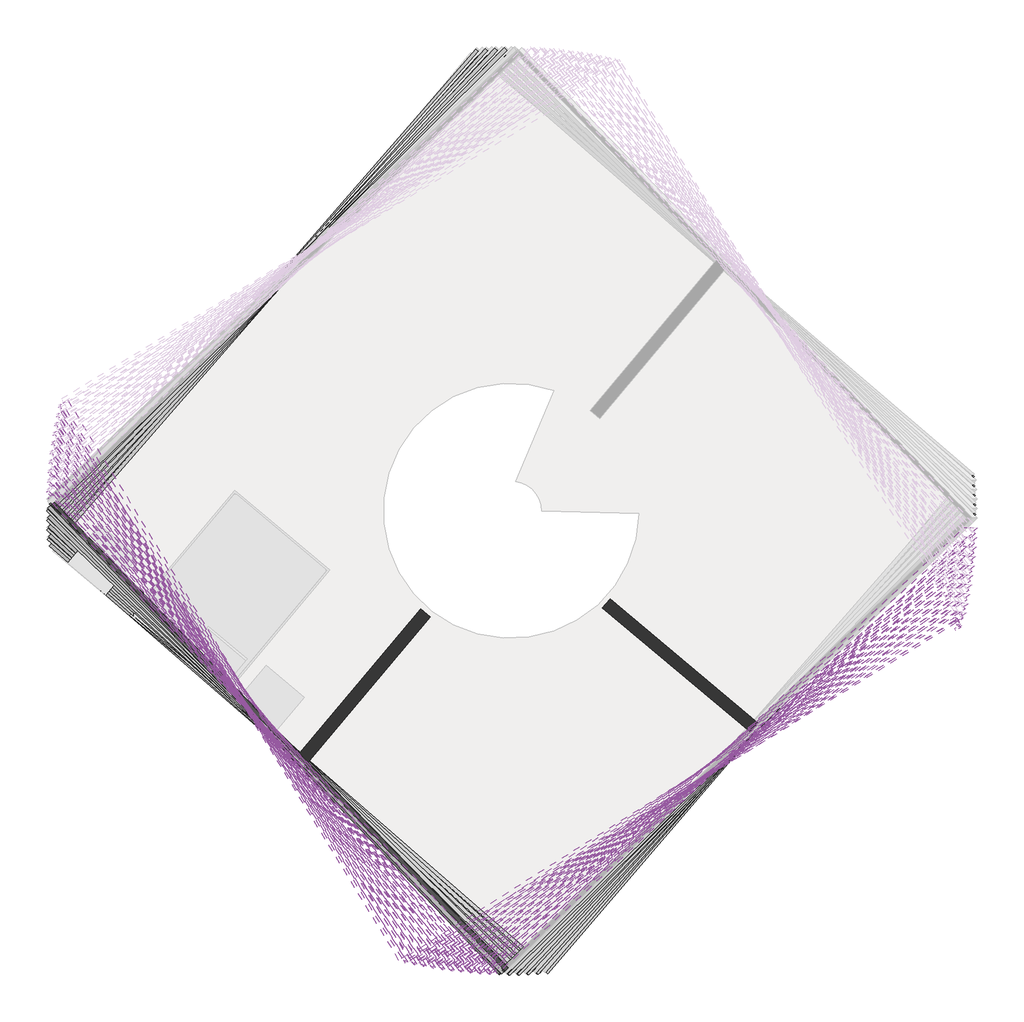
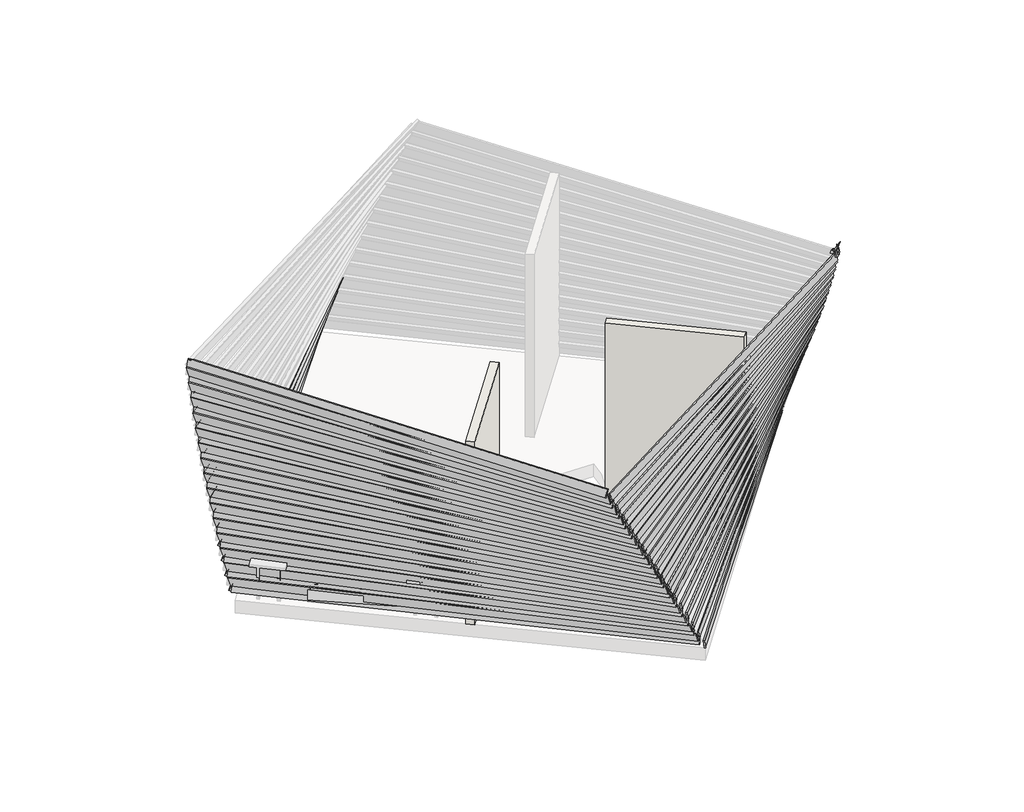
# One storey, part 1 of 2: 33 plates, 32 members, 2 walls.
"""IFC4 building model written with IfcOpenShell, lengths in millimetres."""

import ifcopenshell
import ifcopenshell.guid

model = None  # the IFC model being written
_history = None  # IfcOwnerHistory: only IFC2X3 demands one
_inside = {}  # id of a spatial element -> (the spatial element, [elements in it])
_under = {}  # id of a project, library or spatial element -> (it, [spatial elements below it])
_declared = {}  # id of a project -> (the project, [libraries it declares])
_typed = {}  # id of a type object -> (the type object, [elements of that type])
_made_of = {}  # id of a material, layer set ... -> (it, [elements and type objects made of it])


def new_model(schema):
    """Start an empty IFC model of exactly this schema.

    Asked for "IFC4X3", IfcOpenShell would pick the latest addendum, in which some entities
    have other attributes; the version numbers below select the first issue.
    IFC2X3 requires an IfcOwnerHistory on every rooted entity: one is made here for all.
    """
    global model, _history
    if schema == "IFC4X3":
        model = ifcopenshell.file(schema_version=(4, 3, 0, 0))
    else:
        model = ifcopenshell.file(schema=schema)
    _inside.clear()
    _under.clear()
    _declared.clear()
    _typed.clear()
    _made_of.clear()
    _history = None
    if model.schema == "IFC2X3":
        org = make("IfcOrganization", Name="unknown")
        user = make(
            "IfcPersonAndOrganization",
            ThePerson=make("IfcPerson", FamilyName="unknown"),
            TheOrganization=org,
        )
        app = make(
            "IfcApplication",
            ApplicationDeveloper=org,
            Version="unknown",
            ApplicationFullName="unknown",
            ApplicationIdentifier="unknown",
        )
        _history = make(
            "IfcOwnerHistory",
            OwningUser=user,
            OwningApplication=app,
            ChangeAction="ADDED",
            CreationDate=0,
        )
    return model


def make(cls, **values):
    """One entity of the class cls with the attributes given. An attribute that is None is left unset."""
    return model.create_entity(
        cls, **{name: value for name, value in values.items() if value is not None}
    )


def rooted(cls, **values):
    """An entity with a GlobalId (a new one), such as an element, a storey or a relation."""
    return make(cls, GlobalId=ifcopenshell.guid.new(), OwnerHistory=_history, **values)


def si_unit(unit_type, name, prefix=None):
    """IfcSIUnit, for example si_unit("LENGTHUNIT", "METRE", prefix="MILLI")."""
    return make("IfcSIUnit", UnitType=unit_type, Prefix=prefix, Name=name)


def assignment(units):
    """IfcUnitAssignment: the units of a project."""
    return None if units is None else make("IfcUnitAssignment", Units=units)


def point(xyz):
    """IfcCartesianPoint."""
    return None if xyz is None else make("IfcCartesianPoint", Coordinates=xyz)


def direction(xyz):
    """IfcDirection."""
    return None if xyz is None else make("IfcDirection", DirectionRatios=xyz)


def frame(location, z_axis=None, x_axis=None):
    """IfcAxis2Placement3D, a coordinate frame: its origin and axes. An axis left out is left unset."""
    return make(
        "IfcAxis2Placement3D",
        Location=point(location),
        Axis=direction(z_axis),
        RefDirection=direction(x_axis),
    )


def origin():
    """The frame at (0, 0, 0) with its axes left unset."""
    return frame((0.0, 0.0, 0.0))


def place(relative_to, where):
    """IfcLocalPlacement: puts the frame where relative to a parent placement (None: the world)."""
    return make(
        "IfcLocalPlacement", PlacementRelTo=relative_to, RelativePlacement=where
    )


def context(
    kind, dimensions, precision=None, world=None, true_north=None, identifier=None
):
    """IfcGeometricRepresentationContext, for example the 3D "Model" context."""
    return make(
        "IfcGeometricRepresentationContext",
        ContextIdentifier=identifier,
        ContextType=kind,
        CoordinateSpaceDimension=dimensions,
        Precision=precision,
        WorldCoordinateSystem=world,
        TrueNorth=true_north,
    )


def project(units=None, contexts=None):
    """IfcProject with its units and contexts."""
    return rooted(
        "IfcProject",
        Name="project",
        RepresentationContexts=contexts,
        UnitsInContext=assignment(units),
    )


def spatial(cls, under=None, at=None, **own):
    """A site, building, storey or space (cls), placed at a placement, below another one or the project."""
    s = rooted(cls, ObjectPlacement=at, **own)
    if under is not None:
        _under.setdefault(under.id(), (under, []))[1].append(s)
    return s


def polyline(points):
    """IfcPolyline through the points."""
    return make("IfcPolyline", Points=[point(p) for p in points])


def outline(outer, holes=None, kind="AREA"):
    """IfcArbitraryClosedProfileDef: a profile drawn as a closed curve; with holes, ...WithVoids."""
    if holes is None:
        return make("IfcArbitraryClosedProfileDef", ProfileType=kind, OuterCurve=outer)
    return make(
        "IfcArbitraryProfileDefWithVoids",
        ProfileType=kind,
        OuterCurve=outer,
        InnerCurves=holes,
    )


def extrude(swept, where, along, depth):
    """IfcExtrudedAreaSolid: the profile swept, set in the frame where, extruded along a direction by depth."""
    return make(
        "IfcExtrudedAreaSolid",
        SweptArea=swept,
        Position=where,
        ExtrudedDirection=direction(along),
        Depth=depth,
    )


def faces_of(points, faces, orient=None, outer=None):
    """IfcFace entities. A face is a list of loops; a loop is a list of indices into points, from 0.

    orient and outer hold one flag for each loop. By default every Orientation is true, the
    first loop of a face is its IfcFaceOuterBound and the others are IfcFaceBound.
    """
    made = []
    for i, loops in enumerate(faces):
        bounds = []
        for j, loop in enumerate(loops):
            is_outer = j == 0 if outer is None else outer[i][j]
            bounds.append(
                make(
                    "IfcFaceOuterBound" if is_outer else "IfcFaceBound",
                    Bound=make("IfcPolyLoop", Polygon=[points[k] for k in loop]),
                    Orientation=True if orient is None else orient[i][j],
                )
            )
        made.append(make("IfcFace", Bounds=bounds))
    return made


def faceted_brep(points, faces, orient=None, outer=None, voids=None):
    """IfcFacetedBrep: a solid bounded by flat faces; with voids (closed shells), ...WithVoids."""
    shared = [point(p) for p in points]
    hull = make("IfcClosedShell", CfsFaces=faces_of(shared, faces, orient, outer))
    if voids is None:
        return make("IfcFacetedBrep", Outer=hull)
    return make(
        "IfcFacetedBrepWithVoids",
        Outer=hull,
        Voids=[
            make(cls, CfsFaces=faces_of(shared, fs, o, b)) for cls, fs, o, b in voids
        ],
    )


def shape(context_of_items, identifier, shape_type, items):
    """IfcShapeRepresentation: the items that make up one representation, for example the "Body"."""
    return make(
        "IfcShapeRepresentation",
        ContextOfItems=context_of_items,
        RepresentationIdentifier=identifier,
        RepresentationType=shape_type,
        Items=items,
    )


def source(mapping_origin, context_of_items, identifier, shape_type, items):
    """IfcRepresentationMap: a shape defined once, which mapped items show again and again."""
    return make(
        "IfcRepresentationMap",
        MappingOrigin=mapping_origin,
        MappedRepresentation=shape(context_of_items, identifier, shape_type, items),
    )


def transform(
    local_origin,
    x_axis=None,
    y_axis=None,
    z_axis=None,
    scale=None,
    scale2=None,
    scale3=None,
    uniform=True,
):
    """IfcCartesianTransformationOperator3D, or its non-uniform kind. x_axis, y_axis, z_axis: its Axis1, 2, 3."""
    if uniform:
        return make(
            "IfcCartesianTransformationOperator3D",
            Axis1=direction(x_axis),
            Axis2=direction(y_axis),
            LocalOrigin=point(local_origin),
            Scale=scale,
            Axis3=direction(z_axis),
        )
    return make(
        "IfcCartesianTransformationOperator3DnonUniform",
        Axis1=direction(x_axis),
        Axis2=direction(y_axis),
        LocalOrigin=point(local_origin),
        Scale=scale,
        Axis3=direction(z_axis),
        Scale2=scale2,
        Scale3=scale3,
    )


def mapped(mapping_source, mapping_target):
    """IfcMappedItem: shows the shape of a source again, moved by a transform."""
    return make(
        "IfcMappedItem", MappingSource=mapping_source, MappingTarget=mapping_target
    )


def made_of(thing, what):
    """Note that an element or type object is made of a material, layer set ...; save() writes the relation."""
    if what is not None:
        _made_of.setdefault(what.id(), (what, []))[1].append(thing)
    return thing


def element(
    cls,
    number,
    at=None,
    inside=None,
    cuts=None,
    type_object=None,
    material=None,
    context=None,
    identifier="Body",
    shape_type=None,
    held_by="IfcProductDefinitionShape",
    body=None,
    shapes=None,
    **own,
):
    """One element of the class cls, such as IfcWall. Its Tag is "e" and its number.

    at: its placement. inside: the storey or other place that contains it. cuts: it is an
    opening in that element (IfcRelVoidsElement). A single representation is given by context,
    identifier, shape_type and body (its items); several are given by shapes. held_by: the class
    of the entity that holds the representations. save() writes the other relations.
    """
    e = rooted(cls, Tag="e%d" % number, ObjectPlacement=at, **own)
    if body is not None:
        shapes = [shape(context, identifier, shape_type, body)]
    if shapes is not None:
        e.Representation = make(held_by, Representations=shapes)
    if inside is not None:
        _inside.setdefault(inside.id(), (inside, []))[1].append(e)
    if cuts is not None:
        rooted(
            "IfcRelVoidsElement", RelatingBuildingElement=cuts, RelatedOpeningElement=e
        )
    if type_object is not None:
        _typed.setdefault(type_object.id(), (type_object, []))[1].append(e)
    return made_of(e, material)


def aggregate(whole, parts):
    """IfcRelAggregates: a whole, such as a stair, and the parts it consists of."""
    return rooted("IfcRelAggregates", RelatingObject=whole, RelatedObjects=parts)


def save(model, path):
    """Write the relations noted so far, then the file.

    IfcRelAggregates (storeys below a building ...), IfcRelContainedInSpatialStructure (elements
    in a storey), IfcRelDefinesByType, IfcRelAssociatesMaterial and IfcRelDeclares: one each for
    every whole, place, type object, material and project.
    """
    for whole, parts in _under.values():
        aggregate(whole, parts)
    for where, things in _inside.values():
        rooted(
            "IfcRelContainedInSpatialStructure",
            RelatedElements=things,
            RelatingStructure=where,
        )
    for kind, things in _typed.values():
        rooted("IfcRelDefinesByType", RelatedObjects=things, RelatingType=kind)
    for what, things in _made_of.values():
        rooted("IfcRelAssociatesMaterial", RelatedObjects=things, RelatingMaterial=what)
    for by, libraries in _declared.values():
        rooted("IfcRelDeclares", RelatingContext=by, RelatedDefinitions=libraries)
    model.write(path)


def rectangular_mullion_0e496170(model_context):
    return source(origin(), model_context, "Body", "SweptSolid", [
        extrude(outline(polyline([(-35.3553391, 70.7106781), (70.7106781, -35.3553391), (35.3553391, -70.7106781), (-70.7106781, 35.3553391), (-35.3553391, 70.7106781)])), frame((0.0, 0.0, -8000.0002611), z_axis=(0.0, 0.0, 1.0), x_axis=(1.0, 0.0, 0.0)), (0.0, 0.0, 1.0), 8000.0002611),
    ])


def rectangular_mullion_04c84a83(model_context):
    return source(origin(), model_context, "Body", "SweptSolid", [
        extrude(outline(polyline([(-35.3553391, 70.7106781), (70.7106781, -35.3553391), (35.3553391, -70.7106781), (-70.7106781, 35.3553391), (-35.3553391, 70.7106781)])), frame((0.0, 0.0, -7999.7790849), z_axis=(0.0, 0.0, 1.0), x_axis=(1.0, 0.0, 0.0)), (0.0, 0.0, 1.0), 7999.7790849),
    ])


def rectangular_mullion_5ffb7332(model_context):
    return source(origin(), model_context, "Body", "SweptSolid", [
        extrude(outline(polyline([(-35.3553391, 70.7106781), (70.7106781, -35.3553391), (35.3553391, -70.7106781), (-70.7106781, 35.3553391), (-35.3553391, 70.7106781)])), frame((0.0, 0.0, -7999.4864286), z_axis=(0.0, 0.0, 1.0), x_axis=(1.0, 0.0, 0.0)), (0.0, 0.0, 1.0), 7999.4864286),
    ])


def rectangular_mullion_42344c31(model_context):
    return source(origin(), model_context, "Body", "SweptSolid", [
        extrude(outline(polyline([(-35.3553391, 70.7106781), (70.7106781, -35.3553391), (35.3553391, -70.7106781), (-70.7106781, 35.3553391), (-35.3553391, 70.7106781)])), frame((0.0, 0.0, -7999.2546449), z_axis=(0.0, 0.0, 1.0), x_axis=(1.0, 0.0, 0.0)), (0.0, 0.0, 1.0), 7999.2546449),
    ])


def rectangular_mullion_749d1d03(model_context):
    return source(origin(), model_context, "Body", "Brep", [
        faceted_brep([(-35.3553391, 70.7106781, -7999.1607688), (70.7106781, -35.3553391, -7999.1607688), (35.3553391, -70.7106781, -7999.1607688), (-70.7106781, 35.3553391, -7999.1607688), (-70.7106781, 35.3553391, 10.0516542), (-35.3553391, 70.7106781, 55.0905224), (35.3553391, -70.7106781, -55.0905224), (70.7106781, -35.3553391, -10.0516542)], [[[0, 1, 2, 3]], [[4, 5, 0, 3]], [[6, 4, 3, 2]], [[7, 6, 2, 1]], [[5, 7, 1, 0]], [[5, 4, 6, 7]]]),
    ])


def rectangular_mullion_bea0bdf5(model_context):
    return source(origin(), model_context, "Body", "Brep", [
        faceted_brep([(-35.3553391, 70.7106781, -7999.3358332), (70.7106781, -35.3553391, -7999.3358332), (35.3553391, -70.7106781, -7999.3358332), (-70.7106781, 35.3553391, -7999.3358332), (-70.7106781, 35.3553391, 10.0090632), (-35.3553391, 70.7106781, 55.0597182), (35.3553391, -70.7106781, -55.0597182), (70.7106781, -35.3553391, -10.0090632)], [[[0, 1, 2, 3]], [[4, 5, 0, 3]], [[6, 4, 3, 2]], [[7, 6, 2, 1]], [[5, 7, 1, 0]], [[5, 4, 6, 7]]]),
    ])


def rectangular_mullion_7177dd57(model_context):
    return source(origin(), model_context, "Body", "Brep", [
        faceted_brep([(-35.3553391, 70.7106781, -7999.2401644), (70.7106781, -35.3553391, -7999.2401644), (35.3553391, -70.7106781, -7999.2401644), (-70.7106781, 35.3553391, -7999.2401644), (-70.7106781, 35.3553391, 10.0207535), (-35.3553391, 70.7106781, 55.0681747), (35.3553391, -70.7106781, -55.0681747), (70.7106781, -35.3553391, -10.0207535)], [[[0, 1, 2, 3]], [[4, 5, 0, 3]], [[6, 4, 3, 2]], [[7, 6, 2, 1]], [[5, 7, 1, 0]], [[5, 4, 6, 7]]]),
    ])


def rectangular_mullion_43aaade2(model_context):
    return source(origin(), model_context, "Body", "Brep", [
        faceted_brep([(-35.3553391, 70.7106781, -7999.1801797), (70.7106781, -35.3553391, -7999.1801797), (35.3553391, -70.7106781, -7999.1801797), (-70.7106781, 35.3553391, -7999.1801797), (-70.7106781, 35.3553391, 10.0345933), (-35.3553391, 70.7106781, 55.0781847), (35.3553391, -70.7106781, -55.0781847), (70.7106781, -35.3553391, -10.0345933)], [[[0, 1, 2, 3]], [[4, 5, 0, 3]], [[6, 4, 3, 2]], [[7, 6, 2, 1]], [[5, 7, 1, 0]], [[5, 4, 6, 7]]]),
    ])


def rectangular_mullion_b81ce2a0(model_context):
    return source(origin(), model_context, "Body", "Brep", [
        faceted_brep([(-35.3553391, 70.7106781, -7999.1836632), (70.7106781, -35.3553391, -7999.1836632), (35.3553391, -70.7106781, -7999.1836632), (-70.7106781, 35.3553391, -7999.1836632), (-70.7106781, 35.3553391, 10.0709562), (-35.3553391, 70.7106781, 55.104478), (35.3553391, -70.7106781, -55.104478), (70.7106781, -35.3553391, -10.0709562)], [[[0, 1, 2, 3]], [[4, 5, 0, 3]], [[6, 4, 3, 2]], [[7, 6, 2, 1]], [[5, 7, 1, 0]], [[5, 4, 6, 7]]]),
    ])


def rectangular_mullion_9c5b585c(model_context):
    return source(origin(), model_context, "Body", "Brep", [
        faceted_brep([(-35.3553391, 70.7106781, -7999.2474034), (70.7106781, -35.3553391, -7999.2474034), (35.3553391, -70.7106781, -7999.2474034), (-70.7106781, 35.3553391, -7999.2474034), (-70.7106781, 35.3553391, 10.0945584), (-35.3553391, 70.7106781, 55.1215388), (35.3553391, -70.7106781, -55.1215388), (70.7106781, -35.3553391, -10.0945584)], [[[0, 1, 2, 3]], [[4, 5, 0, 3]], [[6, 4, 3, 2]], [[7, 6, 2, 1]], [[5, 7, 1, 0]], [[5, 4, 6, 7]]]),
    ])


def rectangular_mullion_98a71f57(model_context):
    return source(origin(), model_context, "Body", "Brep", [
        faceted_brep([(-35.3553391, 70.7106781, -7999.3473161), (70.7106781, -35.3553391, -7999.3473161), (35.3553391, -70.7106781, -7999.3473161), (-70.7106781, 35.3553391, -7999.3473161), (-70.7106781, 35.3553391, 10.1224649), (-35.3553391, 70.7106781, 55.1417053), (35.3553391, -70.7106781, -55.1417053), (70.7106781, -35.3553391, -10.1224649)], [[[0, 1, 2, 3]], [[4, 5, 0, 3]], [[6, 4, 3, 2]], [[7, 6, 2, 1]], [[5, 7, 1, 0]], [[5, 4, 6, 7]]]),
    ])


def rectangular_mullion_5539c6e3(model_context):
    return source(origin(), model_context, "Body", "Brep", [
        faceted_brep([(-35.3553391, 70.7106781, -7999.4755006), (70.7106781, -35.3553391, -7999.4755006), (35.3553391, -70.7106781, -7999.4755006), (-70.7106781, 35.3553391, -7999.4755006), (-70.7106781, 35.3553391, 10.1551702), (-35.3553391, 70.7106781, 55.165332), (35.3553391, -70.7106781, -55.165332), (70.7106781, -35.3553391, -10.1551702)], [[[0, 1, 2, 3]], [[4, 5, 0, 3]], [[6, 4, 3, 2]], [[7, 6, 2, 1]], [[5, 7, 1, 0]], [[5, 4, 6, 7]]]),
    ])


def rectangular_mullion_a716d863(model_context):
    return source(origin(), model_context, "Body", "Brep", [
        faceted_brep([(-35.3553391, 70.7106781, -7999.6208242), (70.7106781, -35.3553391, -7999.6208242), (35.3553391, -70.7106781, -7999.6208242), (-70.7106781, 35.3553391, -7999.6208242), (-70.7106781, 35.3553391, 10.1931486), (-35.3553391, 70.7106781, 55.1927576), (35.3553391, -70.7106781, -55.1927576), (70.7106781, -35.3553391, -10.1931486)], [[[0, 1, 2, 3]], [[4, 5, 0, 3]], [[6, 4, 3, 2]], [[7, 6, 2, 1]], [[5, 7, 1, 0]], [[5, 4, 6, 7]]]),
    ])


def rectangular_mullion_345c46c6(model_context):
    return source(origin(), model_context, "Body", "Brep", [
        faceted_brep([(-35.3553391, 70.7106781, -7999.7689278), (70.7106781, -35.3553391, -7999.7689278), (35.3553391, -70.7106781, -7999.7689278), (-70.7106781, 35.3553391, -7999.7689278), (-70.7106781, 35.3553391, 10.2368528), (-35.3553391, 70.7106781, 55.2243041), (35.3553391, -70.7106781, -55.2243041), (70.7106781, -35.3553391, -10.2368528)], [[[0, 1, 2, 3]], [[4, 5, 0, 3]], [[6, 4, 3, 2]], [[7, 6, 2, 1]], [[5, 7, 1, 0]], [[5, 4, 6, 7]]]),
    ])


def rectangular_mullion_ce6685f0(model_context):
    return source(origin(), model_context, "Body", "SweptSolid", [
        extrude(outline(polyline([(-35.3553391, 70.7106781), (70.7106781, -35.3553391), (35.3553391, -70.7106781), (-70.7106781, 35.3553391), (-35.3553391, 70.7106781)])), frame((0.0, 0.0, -55.2367034), z_axis=(0.0, 0.0, 1.0), x_axis=(1.0, 0.0, 0.0)), (0.0, 0.0, 1.0), 55.2367034),
    ])


def rectangular_mullion_5612cd03(model_context):
    return source(origin(), model_context, "Body", "SweptSolid", [
        extrude(outline(polyline([(-35.3553391, 70.7106781), (70.7106781, -35.3553391), (35.3553391, -70.7106781), (-70.7106781, 35.3553391), (-35.3553391, 70.7106781)])), frame((0.0, 0.0, -33.406833), z_axis=(0.0, 0.0, 1.0), x_axis=(1.0, 0.0, 0.0)), (0.0, 0.0, 1.0), 33.406833),
    ])


def system_panel_glazed_9aac2072(model_context):
    return source(origin(), model_context, "Body", "SweptSolid", [
        extrude(outline(polyline([(0.0, -3959.0393549), (35.3553391, -3959.0393549), (35.3553391, 4028.0553276), (234.5588529, 3958.9170456), (199.2035139, 3958.9168202), (199.254446, -4028.0553276), (0.0, -3959.0393549)])), frame((0.0, -49.5, 0.0), z_axis=(0.0, 1.0, 0.0), x_axis=(0.0, 0.0, 1.0)), (0.0, 0.0, 1.0), 25.0),
    ])


def system_panel_glazed_1248680a(model_context):
    return source(origin(), model_context, "Body", "SweptSolid", [
        extrude(outline(polyline([(0.0, -3958.7701168), (35.3553391, -3958.7701168), (35.3553391, 4027.9908618), (234.4800551, 3958.6624486), (199.124716, 3958.6622495), (199.1697072, -4027.9908618), (0.0, -3958.7701168)])), frame((0.0, -49.5, 0.0), z_axis=(0.0, 1.0, 0.0), x_axis=(0.0, 0.0, 1.0)), (0.0, 0.0, 1.0), 25.0),
    ])


def system_panel_glazed_ce91f84a(model_context):
    return source(origin(), model_context, "Body", "SweptSolid", [
        extrude(outline(polyline([(0.0, -3958.544175), (35.3553391, -3958.544175), (35.3553391, 4027.9549227), (234.4222112, 3958.4885806), (199.0668722, 3958.4884774), (199.0901703, -4027.9549227), (0.0, -3958.544175)])), frame((0.0, -49.5, 0.0), z_axis=(0.0, 1.0, 0.0), x_axis=(0.0, 0.0, 1.0)), (0.0, 0.0, 1.0), 25.0),
    ])


def system_panel_glazed_df643311(model_context):
    return source(origin(), model_context, "Body", "SweptSolid", [
        extrude(outline(polyline([(0.0, -3958.3728013), (35.3553391, -3958.3728013), (35.3553391, 4028.0187252), (234.3660482, 3958.4192766), (199.0107092, 3958.4193631), (198.9911695, -4028.0187252), (0.0, -3958.3728013)])), frame((0.0, -49.5, 0.0), z_axis=(0.0, 1.0, 0.0), x_axis=(0.0, 0.0, 1.0)), (0.0, 0.0, 1.0), 25.0),
    ])


def system_panel_glazed_2a14b6e4(model_context):
    return source(origin(), model_context, "Body", "SweptSolid", [
        extrude(outline(polyline([(0.0, -3958.4240501), (35.3553391, -3958.4240501), (35.3553391, 4028.218169), (234.3325301, 3958.5389074), (198.9771911, 3958.5391215), (198.928805, -4028.218169), (0.0, -3958.4240501)])), frame((0.0, -49.5, 0.0), z_axis=(0.0, 1.0, 0.0), x_axis=(0.0, 0.0, 1.0)), (0.0, 0.0, 1.0), 25.0),
    ])


def system_panel_glazed_e03a77ac(model_context):
    return source(origin(), model_context, "Body", "SweptSolid", [
        extrude(outline(polyline([(0.0, -3958.6046047), (35.3553391, -3958.6046047), (35.3553391, 4028.4340057), (234.3037327, 3958.6865343), (198.9483937, 3958.6866872), (198.9138478, -4028.4340057), (0.0, -3958.6046047)])), frame((0.0, -49.5, 0.0), z_axis=(0.0, 1.0, 0.0), x_axis=(0.0, 0.0, 1.0)), (0.0, 0.0, 1.0), 25.0),
    ])


def system_panel_glazed_1e46e190(model_context):
    return source(origin(), model_context, "Body", "SweptSolid", [
        extrude(outline(polyline([(0.0, -3958.6114464), (35.3553391, -3958.6114464), (35.3553391, 4028.3169359), (234.2719876, 3958.4942837), (198.9166485, 3958.4940651), (198.9660296, -4028.3169359), (0.0, -3958.6114464)])), frame((0.0, -49.5, 0.0), z_axis=(0.0, 1.0, 0.0), x_axis=(0.0, 0.0, 1.0)), (0.0, 0.0, 1.0), 25.0),
    ])


def system_panel_glazed_c4fd97ea(model_context):
    return source(origin(), model_context, "Body", "SweptSolid", [
        extrude(outline(polyline([(0.0, -3958.7491356), (35.3553391, -3958.7491356), (35.3553391, 4028.0146093), (234.5559336, 3958.8677682), (199.2005945, 3958.8679874), (199.1510815, -4028.0146093), (0.0, -3958.7491356)])), frame((0.0, -49.5, 0.0), z_axis=(0.0, 1.0, 0.0), x_axis=(0.0, 0.0, 1.0)), (0.0, 0.0, 1.0), 25.0),
    ])


def system_panel_glazed_7537b497(model_context):
    return source(origin(), model_context, "Body", "SweptSolid", [
        extrude(outline(polyline([(0.0, -3959.0229169), (35.3553391, -3959.0229169), (35.3553391, 4028.0764592), (234.64232, 3959.1368322), (199.2869809, 3959.1370419), (199.2396119, -4028.0764592), (0.0, -3959.0229169)])), frame((0.0, -49.5, 0.0), z_axis=(0.0, 1.0, 0.0), x_axis=(0.0, 0.0, 1.0)), (0.0, 0.0, 1.0), 25.0),
    ])


def system_panel_glazed_ea61075c(model_context):
    return source(origin(), model_context, "Body", "SweptSolid", [
        extrude(outline(polyline([(0.0, -3958.7388288), (35.3553391, -3958.7388288), (35.3553391, 4028.1708947), (235.3914127, 3958.6179308), (200.0360737, 3958.6177077), (200.0864778, -4028.1708947), (0.0, -3958.7388288)])), frame((0.0, -49.5, 0.0), z_axis=(0.0, 1.0, 0.0), x_axis=(0.0, 0.0, 1.0)), (0.0, 0.0, 1.0), 25.0),
    ])


def system_panel_glazed_c8b449c2(model_context):
    return source(origin(), model_context, "Body", "SweptSolid", [
        extrude(outline(polyline([(0.0, -3958.4846082), (35.3553391, -3958.4846082), (35.3553391, 4028.1165848), (235.3243648, 3958.401505), (199.9690258, 3958.4013511), (200.0037824, -4028.1165848), (0.0, -3958.4846082)])), frame((0.0, -49.5, 0.0), z_axis=(0.0, 1.0, 0.0), x_axis=(0.0, 0.0, 1.0)), (0.0, 0.0, 1.0), 25.0),
    ])


def system_panel_glazed_b9c8f6ca(model_context):
    return source(origin(), model_context, "Body", "SweptSolid", [
        extrude(outline(polyline([(0.0, -3958.3006839), (35.3553391, -3958.3006839), (35.3553391, 4028.1117128), (235.2758426, 3958.2816454), (199.9205036, 3958.2816101), (199.9284866, -4028.1117128), (0.0, -3958.3006839)])), frame((0.0, -49.5, 0.0), z_axis=(0.0, 1.0, 0.0), x_axis=(0.0, 0.0, 1.0)), (0.0, 0.0, 1.0), 25.0),
    ])


def system_panel_glazed_d027619a(model_context):
    return source(origin(), model_context, "Body", "SweptSolid", [
        extrude(outline(polyline([(0.0, -3958.2331101), (35.3553391, -3958.2331101), (35.3553391, 4028.3015014), (235.2187437, 3958.3356687), (199.8634046, 3958.3358597), (199.8202529, -4028.3015014), (0.0, -3958.2331101)])), frame((0.0, -49.5, 0.0), z_axis=(0.0, 1.0, 0.0), x_axis=(0.0, 0.0, 1.0)), (0.0, 0.0, 1.0), 25.0),
    ])


def system_panel_glazed_ae9a7b9e(model_context):
    return source(origin(), model_context, "Body", "SweptSolid", [
        extrude(outline(polyline([(0.0, -3958.3929013), (35.3553391, -3958.3929013), (35.3553391, 4028.5329041), (235.1902238, 3958.4993271), (199.8348847, 3958.4995256), (199.7900514, -4028.5329041), (0.0, -3958.3929013)])), frame((0.0, -49.5, 0.0), z_axis=(0.0, 1.0, 0.0), x_axis=(0.0, 0.0, 1.0)), (0.0, 0.0, 1.0), 25.0),
    ])


def system_panel_glazed_db2940a7(model_context):
    return source(origin(), model_context, "Body", "SweptSolid", [
        extrude(outline(polyline([(0.0, -3958.4484867), (35.3553391, -3958.4484867), (35.3553391, 4028.4582851), (235.1502568, 3958.3300218), (199.7949178, 3958.329801), (199.8448074, -4028.4582851), (0.0, -3958.4484867)])), frame((0.0, -49.5, 0.0), z_axis=(0.0, 1.0, 0.0), x_axis=(0.0, 0.0, 1.0)), (0.0, 0.0, 1.0), 25.0),
    ])


def system_panel_glazed_81bebace(model_context):
    return source(origin(), model_context, "Body", "SweptSolid", [
        extrude(outline(polyline([(0.0, -3958.4984909), (35.3553391, -3958.4984909), (35.3553391, 4028.1402063), (235.3994701, 3958.60512), (200.0441311, 3958.6053171), (199.9996015, -4028.1402063), (0.0, -3958.4984909)])), frame((0.0, -49.5, 0.0), z_axis=(0.0, 1.0, 0.0), x_axis=(0.0, 0.0, 1.0)), (0.0, 0.0, 1.0), 25.0),
    ])


def system_panel_glazed_1607d224(model_context):
    return source(origin(), model_context, "Body", "SweptSolid", [
        extrude(outline(polyline([(0.0, -3958.7518267), (35.3553391, -3958.7518267), (35.3553391, 4028.204431), (235.485295, 3958.8750513), (200.129956, 3958.8752783), (200.0786736, -4028.204431), (0.0, -3958.7518267)])), frame((0.0, -49.5, 0.0), z_axis=(0.0, 1.0, 0.0), x_axis=(0.0, 0.0, 1.0)), (0.0, 0.0, 1.0), 25.0),
    ])


def system_panel_glazed_255fc0b9(model_context):
    return source(origin(), model_context, "Body", "SweptSolid", [
        extrude(outline(polyline([(0.0, -3956.1046567), (35.3553391, -3956.1046567), (35.3553391, 4031.0223473), (235.5290854, 3961.7982225), (200.1737464, 3961.7984265), (200.1735967, 3935.8556462), (216.0829691, 3932.4976189), (216.0408196, -4031.0223473), (0.0, -3956.1046567)])), frame((0.0, -49.5, 0.0), z_axis=(0.0, 1.0, 0.0), x_axis=(0.0, 0.0, 1.0)), (0.0, 0.0, 1.0), 25.0),
    ])


def system_panel_glazed_d456bf06(model_context):
    return source(origin(), model_context, "Body", "SweptSolid", [
        extrude(outline(polyline([(0.0, 13.3598871), (35.3553391, 13.3598871), (35.3553391, 34.5595931), (235.5726611, -34.5595931), (0.0, 13.3598871)])), frame((0.0, -49.5, 0.0), z_axis=(0.0, 1.0, 0.0), x_axis=(0.0, 0.0, 1.0)), (0.0, 0.0, 1.0), 25.0),
    ])


def system_panel_glazed_54b3e94c(model_context):
    return source(origin(), model_context, "Body", "SweptSolid", [
        extrude(outline(polyline([(0.0, 23.3505759), (35.3553391, 23.3505759), (35.3553391, 58.0717743), (235.5388878, -58.0717743), (0.0, 23.3505759)])), frame((0.0, -49.5, 0.0), z_axis=(0.0, 1.0, 0.0), x_axis=(0.0, 0.0, 1.0)), (0.0, 0.0, 1.0), 25.0),
    ])


model = new_model("IFC4")

# Units and contexts
model_context = context("Model", 3, world=origin())
ifc_project = project(units=[si_unit("LENGTHUNIT", "METRE", prefix="MILLI")], contexts=[model_context])

# Site, building, storey
site = spatial("IfcSite", under=ifc_project)
building = spatial("IfcBuilding", under=site)
storey = spatial("IfcBuildingStorey", under=building, Name="Planta Arquitectonica Nivel 200", Elevation=8000.0)

# Members
placement = place(None, origin())
rectangular_mullion_shape = rectangular_mullion_0e496170(model_context)
element("IfcMember", 1, ObjectType="Rectangular Mullion : tilted mullions", at=placement, inside=storey, context=model_context, shape_type="MappedRepresentation", body=[
    mapped(rectangular_mullion_shape, transform((2975.240903, -5525.8686944, 8204.4589901), x_axis=(-0.21724568349156126, -0.2496700919916238, 0.9436467337776243), y_axis=(-0.6194302128398149, -0.7118815699190423, -0.3309544407177845), z_axis=(0.7543941439496372, -0.6564217208277724, 0.0))),
])
element("IfcMember", 2, ObjectType="Rectangular Mullion : tilted mullions", at=placement, inside=storey, context=model_context, shape_type="MappedRepresentation", body=[
    mapped(rectangular_mullion_shape, transform((2859.2007505, -5532.6680381, 8438.7447875), x_axis=(-0.22224975332135613, -0.24506514731561752, 0.9436885718921106), y_axis=(-0.6339549131651793, -0.6990345404867353, -0.3308351240122925), z_axis=(0.740747065618438, -0.6717840313506073, 0.0))),
])
element("IfcMember", 3, ObjectType="Rectangular Mullion : tilted mullions", at=placement, inside=storey, context=model_context, shape_type="MappedRepresentation", body=[
    mapped(rectangular_mullion_shape, transform((1251.60303, -5380.395406, 11720.5093122), x_axis=(-0.2792878188119162, -0.17036612677950314, 0.9449728552235945), y_axis=(-0.8067260220688225, -0.4921044832415637, -0.3271487473467803), z_axis=(0.5207604435633492, -0.8537028525310806, 0.0))),
])
element("IfcMember", 4, ObjectType="Rectangular Mullion : tilted mullions", at=placement, inside=storey, context=model_context, shape_type="MappedRepresentation", body=[
    mapped(rectangular_mullion_shape, transform((-3059.8910049, -274.5134126, 8204.4589901), x_axis=(-0.24967009199163023, 0.21724568349156653, 0.9436467337776214), y_axis=(-0.7118815699190397, 0.6194302128398134, -0.3309544407177928), z_axis=(-0.6564217208277727, -0.754394143949637, 0.0))),
])
element("IfcMember", 5, ObjectType="Rectangular Mullion : tilted mullions", at=placement, inside=storey, context=model_context, shape_type="MappedRepresentation", body=[
    mapped(rectangular_mullion_shape, transform((-3066.6903485, -158.4732601, 8438.7447875), x_axis=(-0.2450651473156227, 0.22224975332136054, 0.9436885718921082), y_axis=(-0.6990345404867332, 0.6339549131651782, -0.3308351240122993), z_axis=(-0.6717840313506076, -0.7407470656184376, 0.0))),
])
rectangular_mullion_2_shape = rectangular_mullion_04c84a83(model_context)
element("IfcMember", 6, ObjectType="Rectangular Mullion : tilted mullions", at=placement, inside=storey, context=model_context, shape_type="MappedRepresentation", body=[
    mapped(rectangular_mullion_2_shape, transform((2743.0608469, -5537.0550323, 8673.0346683), x_axis=(-0.22716322400261674, -0.24036856712439816, 0.943726560821142), y_axis=(-0.6482087487706546, -0.6858901075365376, -0.3307267427963746), z_axis=(0.7267890255623838, -0.6868607663290142, 0.0))),
])
element("IfcMember", 7, ObjectType="Rectangular Mullion : tilted mullions", at=placement, inside=storey, context=model_context, shape_type="MappedRepresentation", body=[
    mapped(rectangular_mullion_2_shape, transform((1363.5523833, -5406.2133058, 11485.8904822), x_axis=(-0.27626315380177624, -0.1763175978064715, 0.9447702231523026), y_axis=(-0.7963947160812201, -0.5082777102659177, -0.32773346708071865), z_axis=(0.5379908233877311, -0.842950694851479, 0.0))),
])
element("IfcMember", 8, ObjectType="Rectangular Mullion : tilted mullions", at=placement, inside=storey, context=model_context, shape_type="MappedRepresentation", body=[
    mapped(rectangular_mullion_2_shape, transform((-3071.0773427, -42.3333565, 8673.0346683), x_axis=(-0.24036856712440186, 0.22716322400261998, 0.9437265608211404), y_axis=(-0.6858901075365361, 0.6482087487706536, -0.3307267427963795), z_axis=(-0.6868607663290143, -0.7267890255623836, 0.0))),
])
rectangular_mullion_3_shape = rectangular_mullion_5ffb7332(model_context)
element("IfcMember", 9, ObjectType="Rectangular Mullion : tilted mullions", at=placement, inside=storey, context=model_context, shape_type="MappedRepresentation", body=[
    mapped(rectangular_mullion_3_shape, transform((2626.8816383, -5539.0428385, 8907.3311201), x_axis=(-0.23197908200136044, -0.23557716819595317, 0.9437632665762012), y_axis=(-0.6621862623905888, -0.6724570300322276, -0.33062198454037856), z_axis=(0.7125272341566943, -0.7016444545387724, 0.0))),
])
element("IfcMember", 10, ObjectType="Rectangular Mullion : tilted mullions", at=placement, inside=storey, context=model_context, shape_type="MappedRepresentation", body=[
    mapped(rectangular_mullion_3_shape, transform((2510.7234794, -5538.6445168, 9141.6368322), x_axis=(-0.23668996190483846, -0.23068834343080663, 0.9438012238488762), y_axis=(-0.6758822191149877, -0.6587442417378965, -0.3305136152435534), z_axis=(0.6979692599374888, -0.7161277205794466, 0.0))),
])
element("IfcMember", 11, ObjectType="Rectangular Mullion : tilted mullions", at=placement, inside=storey, context=model_context, shape_type="MappedRepresentation", body=[
    mapped(rectangular_mullion_3_shape, transform((2394.6466542, -5535.873018, 9375.9546695), x_axis=(-0.2412881999686787, -0.2257000879375215, 0.943842929125853), y_axis=(-0.6892916254182386, -0.6447608316183239, -0.33039449925676734), z_axis=(0.6831230194365855, -0.730303320761889, 0.0))),
])
element("IfcMember", 12, ObjectType="Rectangular Mullion : tilted mullions", at=placement, inside=storey, context=model_context, shape_type="MappedRepresentation", body=[
    mapped(rectangular_mullion_3_shape, transform((1703.2656415, -5470.117416, 10782.2929124), x_axis=(-0.26605941973851915, -0.19365043540492372, 0.9443049793556559), y_axis=(-0.7634850553518003, -0.5556999768673239, -0.3290715818239461), z_axis=(0.588475110283231, -0.8085153335448495, 0.0))),
])
element("IfcMember", 13, ObjectType="Rectangular Mullion : tilted mullions", at=placement, inside=storey, context=model_context, shape_type="MappedRepresentation", body=[
    mapped(rectangular_mullion_3_shape, transform((1589.4442885, -5451.0860952, 11016.7856859), x_axis=(-0.26964124833447933, -0.18796383488464596, 0.9444380307738995), y_axis=(-0.7747720193376094, -0.5400847267083234, -0.3286895283210568), z_axis=(0.5718582999731199, -0.8203524149728904, 0.0))),
])
element("IfcMember", 14, ObjectType="Rectangular Mullion : tilted mullions", at=placement, inside=storey, context=model_context, shape_type="MappedRepresentation", body=[
    mapped(rectangular_mullion_3_shape, transform((1476.1863571, -5429.7807783, 11251.3170666), x_axis=(-0.27304510361470985, -0.18218496105086326, 0.9445925107467917), y_axis=(-0.7857426930534145, -0.5242741951232156, -0.328245317774789), z_axis=(0.5550268387251197, -0.831832440035131, 0.0))),
])
element("IfcMember", 15, ObjectType="Rectangular Mullion : tilted mullions", at=placement, inside=storey, context=model_context, shape_type="MappedRepresentation", body=[
    mapped(rectangular_mullion_3_shape, transform((-3073.0651489, 73.8458522, 8907.3311201), x_axis=(-0.23557716819595564, 0.23197908200136308, 0.9437632665761999), y_axis=(-0.6724570300322261, 0.6621862623905884, -0.33062198454038216), z_axis=(-0.701644454538773, -0.7125272341566937, 0.0))),
])
rectangular_mullion_4_shape = rectangular_mullion_42344c31(model_context)
element("IfcMember", 16, ObjectType="Rectangular Mullion : tilted mullions", at=placement, inside=storey, context=model_context, shape_type="MappedRepresentation", body=[
    mapped(rectangular_mullion_4_shape, transform((2278.7113945, -5530.7411769, 9610.2876489), x_axis=(-0.24576588912529984, -0.22061102026629906, 0.9438908334545439), y_axis=(-0.7024097461708791, -0.6305160219722215, -0.33025761841399903), z_axis=(0.6679967636348338, -0.7441641779697461, 0.0))),
])
element("IfcMember", 17, ObjectType="Rectangular Mullion : tilted mullions", at=placement, inside=storey, context=model_context, shape_type="MappedRepresentation", body=[
    mapped(rectangular_mullion_4_shape, transform((2162.9779022, -5523.2617072, 9844.638913), x_axis=(-0.2501149349597387, -0.21542039882177647, 0.9439473349088668), y_axis=(-0.715232119129968, -0.6160191448700338, -0.330096090431934), z_axis=(0.652599061503264, -0.7577034148828017, 0.0))),
])
element("IfcMember", 18, ObjectType="Rectangular Mullion : tilted mullions", at=placement, inside=storey, context=model_context, shape_type="MappedRepresentation", body=[
    mapped(rectangular_mullion_4_shape, transform((2047.5063671, -5513.447198, 10079.0117097), x_axis=(-0.2543271124462252, -0.21012813319745363, 0.9440147708133164), y_axis=(-0.7277545672984731, -0.6012796165594929, -0.3299031865355073), z_axis=(0.6369387801437258, -0.7709143858749962, 0.0))),
])
element("IfcMember", 19, ObjectType="Rectangular Mullion : tilted mullions", at=placement, inside=storey, context=model_context, shape_type="MappedRepresentation", body=[
    mapped(rectangular_mullion_4_shape, transform((1932.3569873, -5501.3101114, 10313.4093713), x_axis=(-0.25839412289397046, -0.20473479058680696, 0.9440954097850662), y_axis=(-0.7399732085805416, -0.5863069105513344, -0.3296723482835162), z_axis=(0.6210250621648647, -0.7837907068619313, 0.0))),
])
element("IfcMember", 20, ObjectType="Rectangular Mullion : tilted mullions", at=placement, inside=storey, context=model_context, shape_type="MappedRepresentation", body=[
    mapped(rectangular_mullion_4_shape, transform((1817.5899879, -5486.8627818, 10547.835293), x_axis=(-0.26230765073129403, -0.19924159728948973, 0.9441914436582035), y_axis=(-0.7518844627065218, -0.5711105295981569, -0.32939720357440455), z_axis=(0.6048673004125406, -0.7963262829341033, 0.0))),
])
rectangular_mullion_5_shape = rectangular_mullion_749d1d03(model_context)
element("IfcMember", 21, ObjectType="Rectangular Mullion : tilted mullions", at=placement, inside=storey, context=model_context, shape_type="MappedRepresentation", body=[
    mapped(rectangular_mullion_5_shape, transform((8212.3768845, -437.0364942, 10116.7536384), x_axis=(0.20926647788558933, -0.25499202272997784, 0.9440268055396704), y_axis=(0.5988841509311498, -0.7297426829649686, -0.32986874726558346), z_axis=(0.7730105529660226, 0.6343931627966714, 0.0))),
])
rectangular_mullion_6_shape = rectangular_mullion_bea0bdf5(model_context)
element("IfcMember", 22, ObjectType="Rectangular Mullion : tilted mullions", at=placement, inside=storey, context=model_context, shape_type="MappedRepresentation", body=[
    mapped(rectangular_mullion_6_shape, transform((8235.9817967, -88.7074569, 9411.054357), x_axis=(0.22494424145595174, -0.24196678466971486, 0.9438496508196664), y_axis=(0.6426435205484025, -0.6912752482546743, -0.33037529666667526), z_axis=(0.7323997499541912, 0.680874882975601, 0.0))),
])
rectangular_mullion_7_shape = rectangular_mullion_7177dd57(model_context)
element("IfcMember", 23, ObjectType="Rectangular Mullion : tilted mullions", at=placement, inside=storey, context=model_context, shape_type="MappedRepresentation", body=[
    mapped(rectangular_mullion_7_shape, transform((8230.4725441, -205.0500189, 9646.2674354), x_axis=(0.21982068854730832, -0.24644218228663103, 0.9438988906002541), y_axis=(0.6283063932047389, -0.7043977512275591, -0.33023458983518034), z_axis=(0.7462639889105191, 0.6656501024227073, 0.0))),
])
rectangular_mullion_8_shape = rectangular_mullion_43aaade2(model_context)
element("IfcMember", 24, ObjectType="Rectangular Mullion : tilted mullions", at=placement, inside=storey, context=model_context, shape_type="MappedRepresentation", body=[
    mapped(rectangular_mullion_8_shape, transform((8222.6000029, -321.1799874, 9881.4994291), x_axis=(0.21459476348816953, -0.25078670599127106, 0.9439571577044714), y_axis=(0.6137167589454584, -0.7172216222137942, -0.330067999688694), z_axis=(0.7598031503441787, 0.6501531917379636, 0.0))),
])
rectangular_mullion_9_shape = rectangular_mullion_b81ce2a0(model_context)
element("IfcMember", 25, ObjectType="Rectangular Mullion : tilted mullions", at=placement, inside=storey, context=model_context, shape_type="MappedRepresentation", body=[
    mapped(rectangular_mullion_9_shape, transform((8199.8157709, -552.5586605, 10352.0334461), x_axis=(0.2038365114020308, -0.25904973376633345, 0.94411011648803), y_axis=(0.583818156005435, -0.7419570558822495, -0.3296302291128022), z_axis=(0.785879785551113, 0.6183793032291236, 0.0))),
])
rectangular_mullion_10_shape = rectangular_mullion_9c5b585c(model_context)
element("IfcMember", 26, ObjectType="Rectangular Mullion : tilted mullions", at=placement, inside=storey, context=model_context, shape_type="MappedRepresentation", body=[
    mapped(rectangular_mullion_10_shape, transform((8184.9291144, -667.6855757, 10587.3422954), x_axis=(0.19830621252374922, -0.262951432455398, 0.944209293665414), y_axis=(0.5685283860545804, -0.7538611705707583, -0.3293460334600375), z_axis=(0.798404734658218, 0.6021211503305132, 0.0))),
])
rectangular_mullion_11_shape = rectangular_mullion_98a71f57(model_context)
element("IfcMember", 27, ObjectType="Rectangular Mullion : tilted mullions", at=placement, inside=storey, context=model_context, shape_type="MappedRepresentation", body=[
    mapped(rectangular_mullion_11_shape, transform((8167.7292382, -782.3562778, 10822.6836672), x_axis=(0.19267759442530746, -0.26668876139791503, 0.9443264526372872), y_axis=(0.553024448586864, -0.7654517675305987, -0.32900995554766627), z_axis=(0.8105796098297019, 0.5856284625326267, 0.0))),
])
rectangular_mullion_12_shape = rectangular_mullion_5539c6e3(model_context)
element("IfcMember", 28, ObjectType="Rectangular Mullion : tilted mullions", at=placement, inside=storey, context=model_context, shape_type="MappedRepresentation", body=[
    mapped(rectangular_mullion_12_shape, transform((8148.2283383, -896.5097321, 11058.0610578), x_axis=(0.18695332607112544, -0.2702534685971306, 0.9444636131594288), y_axis=(0.5373159168274168, -0.7767258989541135, -0.32861601211419506), z_axis=(0.8223989660711255, 0.5689111886798712, 0.0))),
])
rectangular_mullion_13_shape = rectangular_mullion_a716d863(model_context)
element("IfcMember", 29, ObjectType="Rectangular Mullion : tilted mullions", at=placement, inside=storey, context=model_context, shape_type="MappedRepresentation", body=[
    mapped(rectangular_mullion_13_shape, transform((8126.4384873, -1010.0848112, 11293.4779561), x_axis=(0.1811367187333737, -0.2736374622645363, 0.9446226910105067), y_axis=(0.5214122996126669, -0.7876809266349932, -0.32815845506107083), z_axis=(0.8338577234391592, 0.5519794353604697, 0.0))),
])
rectangular_mullion_14_shape = rectangular_mullion_345c46c6(model_context)
element("IfcMember", 30, ObjectType="Rectangular Mullion : tilted mullions", at=placement, inside=storey, context=model_context, shape_type="MappedRepresentation", body=[
    mapped(rectangular_mullion_14_shape, transform((8102.3716385, -1123.020275, 11528.937821), x_axis=(0.17523170814593014, -0.27683286394599926, 0.9448054899817822), y_axis=(0.5053230113678412, -0.7983145170181062, -0.32763178432545975), z_axis=(0.8449511835854164, 0.5348434325647121, 0.0))),
])
rectangular_mullion_15_shape = rectangular_mullion_ce6685f0(model_context)
element("IfcMember", 31, ObjectType="Rectangular Mullion : tilted mullions", at=placement, inside=storey, context=model_context, shape_type="MappedRepresentation", body=[
    mapped(rectangular_mullion_15_shape, transform((8047.4538932, -1187.9900824, 11764.4440588), x_axis=(-0.2760085981890653, -0.16693039753770186, 0.946548200623514), y_axis=(0.8099376723952636, 0.4898514702831408, 0.3225624031042491), z_axis=(-0.5175134979501983, 0.8556750431322337, 0.0))),
])
rectangular_mullion_16_shape = rectangular_mullion_5612cd03(model_context)
element("IfcMember", 32, ObjectType="Rectangular Mullion : tilted mullions", at=placement, inside=storey, context=model_context, shape_type="MappedRepresentation", body=[
    mapped(rectangular_mullion_16_shape, transform((8076.0396328, -1235.254751, 11764.4440588), x_axis=(0.16924283254707925, -0.27983205967217484, 0.94501369408653), y_axis=(0.48905734243752824, -0.8086246334480616, -0.32703076000420866), z_axis=(0.8556750431322533, 0.517513497950166, 0.0))),
])

# Plates
system_panel_glazed_shape = system_panel_glazed_9aac2072(model_context)
element("IfcPlate", 33, ObjectType="System Panel : Glazed", at=placement, inside=storey, context=model_context, shape_type="MappedRepresentation", body=[
    mapped(system_panel_glazed_shape, transform((-766.0575805, -2068.5283174, 11251.3171975), x_axis=(0.5465370261593958, -0.8374349401753602, -3.214763573030216e-06), y_axis=(0.8374348989141635, 0.546536998017806, 0.0003160352982295529), z_axis=(-0.0002629020138336268, -0.0001754171472635911, 0.9999999500556765))),
])
system_panel_glazed_2_shape = system_panel_glazed_1248680a(model_context)
element("IfcPlate", 34, ObjectType="System Panel : Glazed", at=placement, inside=storey, context=model_context, shape_type="MappedRepresentation", body=[
    mapped(system_panel_glazed_2_shape, transform((-674.1214469, -2203.0797802, 10782.2930221), x_axis=(0.5801968296077754, -0.8144762973259966, -2.687162329784578e-06), y_axis=(0.8144762694839222, 0.5801968089052664, 0.0002634078578204674), z_axis=(-0.00021298037371543532, -0.0001550170339510715, 0.9999999653045392))),
])
system_panel_glazed_3_shape = system_panel_glazed_ce91f84a(model_context)
element("IfcPlate", 35, ObjectType="System Panel : Glazed", at=placement, inside=storey, context=model_context, shape_type="MappedRepresentation", body=[
    mapped(system_panel_glazed_3_shape, transform((-420.0945963, -2523.5784249, 9610.28759), x_axis=(0.6603326457249373, -0.7509732332033154, 1.436406563527974e-06), y_axis=(0.750973225966357, 0.6603326390934783, -0.00014010540830437985), z_axis=(0.00010426690532670512, 9.359487781681557e-05, 0.9999999901842056))),
])
element("IfcPlate", 36, ObjectType="System Panel : Glazed", at=placement, inside=storey, context=model_context, shape_type="MappedRepresentation", body=[
    mapped(system_panel_glazed_3_shape, transform((-473.5694613, -2461.442063, 9844.6388898), x_axis=(0.6448027683765851, -0.7643489974439492, 5.670738617925266e-07), y_axis=(0.7643489962933546, 0.6448027673648801, -5.535281176778237e-05), z_axis=(4.194321538502398e-05, 3.6125088602379405e-05, 0.9999999984678724))),
])
element("IfcPlate", 37, ObjectType="System Panel : Glazed", at=placement, inside=storey, context=model_context, shape_type="MappedRepresentation", body=[
    mapped(system_panel_glazed_3_shape, transform((-525.7332269, -2398.286819, 10079.011724), x_axis=(0.6290148623518959, -0.7773932743086371, -3.4901846831708545e-07), y_axis=(0.7773932738642524, 0.6290148619770208, 3.409764140850055e-05), z_axis=(-2.62877392970801e-05, -2.1719247826816377e-05, 0.9999999994186146))),
])
element("IfcPlate", 38, ObjectType="System Panel : Glazed", at=placement, inside=storey, context=model_context, shape_type="MappedRepresentation", body=[
    mapped(system_panel_glazed_3_shape, transform((-576.5622491, -2334.149922, 10313.4094221), x_axis=(0.6129781979723891, -0.7900998220535035, -1.2428862042755527e-06), y_axis=(0.7900998163105476, 0.6129781933256677, 0.00012154521510080989), z_axis=(-9.527099068259847e-05, -7.548657108635388e-05, 0.999999992612608))),
])
element("IfcPlate", 39, ObjectType="System Panel : Glazed", at=placement, inside=storey, context=model_context, shape_type="MappedRepresentation", body=[
    mapped(system_panel_glazed_3_shape, transform((-626.0328782, -2269.0685391, 10547.8353766), x_axis=(0.596702282142663, -0.8024627009908651, -2.0453140470901204e-06), y_axis=(0.802462685148996, 0.5967022698524533, 0.0002002408388942445), z_axis=(-0.00015946536089329235, -0.0001211254537485579, 0.9999999799497115))),
])
system_panel_glazed_4_shape = system_panel_glazed_df643311(model_context)
element("IfcPlate", 40, ObjectType="System Panel : Glazed", at=placement, inside=storey, context=model_context, shape_type="MappedRepresentation", body=[
    mapped(system_panel_glazed_4_shape, transform((-309.3061801, -2644.6452607, 9141.6367189), x_axis=(0.6905825725391471, -0.723253558924936, 2.761832172569364e-06), y_axis=(0.7232535332575958, 0.690582547003742, -0.0002690803383907105), z_axis=(0.00019270603928167766, 0.0001878196971826364, 0.9999999637940713))),
])
element("IfcPlate", 41, ObjectType="System Panel : Glazed", at=placement, inside=storey, context=model_context, shape_type="MappedRepresentation", body=[
    mapped(system_panel_glazed_4_shape, transform((-365.3322807, -2584.6586111, 9375.9545796), x_axis=(0.6755954871658616, -0.73727249895566, 2.1905309621769514e-06), y_axis=(0.7372724824656735, 0.675595471420935, -0.00021352851815625623), z_axis=(0.00015594879138130794, 0.00014587392144798256, 0.9999999772003865))),
])
system_panel_glazed_5_shape = system_panel_glazed_2a14b6e4(model_context)
element("IfcPlate", 42, ObjectType="System Panel : Glazed", at=placement, inside=storey, context=model_context, shape_type="MappedRepresentation", body=[
    mapped(system_panel_glazed_5_shape, transform((-252.0399875, -2703.5009443, 8907.3309935), x_axis=(0.7052854900341087, -0.708923393278736, 3.083817311817699e-06), y_axis=(0.7089233619636472, 0.7052854575732825, -0.00030032949443990086), z_axis=(0.00021073563279618403, 0.00021400422479411708, 0.9999999548963415))),
])
system_panel_glazed_6_shape = system_panel_glazed_e03a77ac(model_context)
element("IfcPlate", 43, ObjectType="System Panel : Glazed", at=placement, inside=storey, context=model_context, shape_type="MappedRepresentation", body=[
    mapped(system_panel_glazed_6_shape, transform((-73.0384546, -2872.9068648, 8204.4589116), x_axis=(0.7476101024060612, -0.6641378883761604, 1.911421881186175e-06), y_axis=(0.6641378771511622, 0.7476100892348428, -0.00018603069108320364), z_axis=(0.00012212103206599764, 0.00014034787168189548, 0.9999999826944641))),
])
element("IfcPlate", 44, ObjectType="System Panel : Glazed", at=placement, inside=storey, context=model_context, shape_type="MappedRepresentation", body=[
    mapped(system_panel_glazed_6_shape, transform((-133.8823087, -2817.6693495, 8438.7446758), x_axis=(0.7338068219099178, -0.6793581883741905, 2.721108122063512e-06), y_axis=(0.6793581650752506, 0.733806795682726, -0.00026486872000857986), z_axis=(0.0001779439661502618, 0.0001962110806736202, 0.9999999649185778))),
])
system_panel_glazed_7_shape = system_panel_glazed_1e46e190(model_context)
element("IfcPlate", 45, ObjectType="System Panel : Glazed", at=placement, inside=storey, context=model_context, shape_type="MappedRepresentation", body=[
    mapped(system_panel_glazed_7_shape, transform((-193.5574356, -2761.1881634, 8673.0345414), x_axis=(0.7196961543845368, -0.6942891655171873, 3.091389998425502e-06), y_axis=(0.6942891347436153, 0.7196961211447066, -0.0003009754570622143), z_axis=(0.0002067391375340664, 0.0002187571974989658, 0.9999999547021079))),
])
system_panel_glazed_8_shape = system_panel_glazed_c4fd97ea(model_context)
element("IfcPlate", 46, ObjectType="System Panel : Glazed", at=placement, inside=storey, context=model_context, shape_type="MappedRepresentation", body=[
    mapped(system_panel_glazed_8_shape, transform((-720.8042595, -2136.2207027, 11016.7858123), x_axis=(0.5634717321852033, -0.8261353442497172, -3.099671963705619e-06), y_axis=(0.8261353065450403, 0.563471705326851, 0.00030426268702787716), z_axis=(-0.00024961558224277625, -0.00017400417174684733, 0.9999999537073037))),
])
system_panel_glazed_9_shape = system_panel_glazed_7537b497(model_context)
element("IfcPlate", 47, ObjectType="System Panel : Glazed", at=placement, inside=storey, context=model_context, shape_type="MappedRepresentation", body=[
    mapped(system_panel_glazed_9_shape, transform((-809.8576245, -2000.0395954, 11485.8906027), x_axis=(0.5294028581355923, -0.848370563957209, -2.9653268296864334e-06), y_axis=(0.848370528254194, 0.5294028348354883, 0.00029198946657629825), z_axis=(-0.00024614541599904903, -0.0001570957540399267, 0.9999999573666783))),
])
system_panel_glazed_10_shape = system_panel_glazed_ea61075c(model_context)
element("IfcPlate", 48, ObjectType="System Panel : Glazed", at=placement, inside=storey, context=model_context, shape_type="MappedRepresentation", body=[
    mapped(system_panel_glazed_10_shape, transform((4824.9662716, -3194.935232, 11058.0611869), x_axis=(0.8281716680412741, 0.5604745206017634, -3.155509541419171e-06), y_axis=(-0.5604744930980834, 0.8281716291389446, 0.0003086677712029972), z_axis=(0.0001756137245678952, -0.00025386132033707547, 0.9999999523571238))),
])
system_panel_glazed_11_shape = system_panel_glazed_c8b449c2(model_context)
element("IfcPlate", 49, ObjectType="System Panel : Glazed", at=placement, inside=storey, context=model_context, shape_type="MappedRepresentation", body=[
    mapped(system_panel_glazed_11_shape, transform((5024.0957785, -3050.8774617, 10352.0335032), x_axis=(0.7921839947117726, 0.6102823268951562, -1.389977621513006e-06), y_axis=(-0.6102823211485512, 0.7921839875608188, 0.00013544658419016207), z_axis=(8.376177458440326e-05, -0.0001064503373646255, 0.9999999908261454))),
])
element("IfcPlate", 50, ObjectType="System Panel : Glazed", at=placement, inside=storey, context=model_context, shape_type="MappedRepresentation", body=[
    mapped(system_panel_glazed_11_shape, transform((4958.614595, -3100.3012041, 10587.3423847), x_axis=(0.8045344729218159, 0.593905953729781, -2.175994068843116e-06), y_axis=(-0.5939059399776303, 0.8045344550702477, 0.00021228308239324643), z_axis=(0.0001278268487118715, -0.00016949672200062692, 0.9999999774655788))),
])
system_panel_glazed_12_shape = system_panel_glazed_b9c8f6ca(model_context)
element("IfcPlate", 51, ObjectType="System Panel : Glazed", at=placement, inside=storey, context=model_context, shape_type="MappedRepresentation", body=[
    mapped(system_panel_glazed_12_shape, transform((5276.1910705, -2839.6960523, 9411.0542708), x_axis=(0.7393710164161282, 0.6732982252162829, 2.094020788909432e-06), y_axis=(-0.6732982109783205, 0.7393710014134733, -0.00020337706541133507), z_axis=(-0.00013848167543882437, 0.00014896120711798409, 0.999999979316692))),
])
element("IfcPlate", 52, ObjectType="System Panel : Glazed", at=placement, inside=storey, context=model_context, shape_type="MappedRepresentation", body=[
    mapped(system_panel_glazed_12_shape, transform((5214.7169508, -2894.4665437, 9646.2673814), x_axis=(0.7530734075428197, 0.6579365036613525, 1.3120076293726281e-06), y_axis=(-0.6579364981874808, 0.7530734015316988, -0.00012750792996446257), z_axis=(-8.488015967820229e-05, 9.515961360180435e-05, 0.9999999918700033))),
])
element("IfcPlate", 53, ObjectType="System Panel : Glazed", at=placement, inside=storey, context=model_context, shape_type="MappedRepresentation", body=[
    mapped(system_panel_glazed_12_shape, transform((5152.1845679, -2947.9362177, 9881.4994117), x_axis=(0.7664473527855179, 0.6423071347944782, 4.241972933370999e-07), y_axis=(-0.642307134234466, 0.7664473521445181, -4.1257298200675404e-05), z_axis=(-2.6824981888902297e-05, 3.134908204115701e-05, 0.9999999991488278))),
])
element("IfcPlate", 54, ObjectType="System Panel : Glazed", at=placement, inside=storey, context=model_context, shape_type="MappedRepresentation", body=[
    mapped(system_panel_glazed_12_shape, transform((5088.6316297, -3000.0811603, 10116.753659), x_axis=(0.7794863033673641, 0.6264192708262031, -4.998250456661352e-07), y_axis=(-0.6264192700658283, 0.779486302460013, 4.865606052843445e-05), z_axis=(3.0868700734220706e-05, -3.761363271746128e-05, 0.999999998816169))),
])
system_panel_glazed_13_shape = system_panel_glazed_d027619a(model_context)
element("IfcPlate", 55, ObjectType="System Panel : Glazed", at=placement, inside=storey, context=model_context, shape_type="MappedRepresentation", body=[
    mapped(system_panel_glazed_13_shape, transform((5395.8133475, -2726.3483609, 8940.6721663), x_axis=(0.711008337036863, 0.7031835782032105, 3.066625593398121e-06), y_axis=(-0.7031835464278617, 0.7110083062055913, -0.0002975563672603938), z_axis=(-0.000211417147316241, 0.00020940865720021047, 0.9999999557254011))),
])
element("IfcPlate", 56, ObjectType="System Panel : Glazed", at=placement, inside=storey, context=model_context, shape_type="MappedRepresentation", body=[
    mapped(system_panel_glazed_13_shape, transform((5336.5691512, -2783.6486725, 9175.8568875), x_axis=(0.7253469834843463, 0.6883834349712823, 2.701454431063291e-06), y_axis=(-0.6883834107910568, 0.7253469590348319, -0.0002622338520532769), z_axis=(-0.00018247693159872873, 0.00018835089713897278, 0.999999965613054))),
])
system_panel_glazed_14_shape = system_panel_glazed_ae9a7b9e(model_context)
element("IfcPlate", 57, ObjectType="System Panel : Glazed", at=placement, inside=storey, context=model_context, shape_type="MappedRepresentation", body=[
    mapped(system_panel_glazed_14_shape, transform((5620.6919191, -2485.0985354, 8000.0043234), x_axis=(0.6506541350675407, 0.759374213756869, 8.04864712566377e-07), y_axis=(-0.7593742114040074, 0.6506541331342522, -7.803753421654452e-05), z_axis=(-5.9783379741058484e-05, 5.016425082207738e-05, 0.9999999969547478))),
])
element("IfcPlate", 58, ObjectType="System Panel : Glazed", at=placement, inside=storey, context=model_context, shape_type="MappedRepresentation", body=[
    mapped(system_panel_glazed_14_shape, transform((5566.3631183, -2547.1700547, 8235.165708), x_axis=(0.666177657626583, 0.7457930869047661, 2.0540501816464792e-06), y_axis=(-0.7457930718416603, 0.6661776447200518, -0.00019916883452603083), z_axis=(-0.00014990710222853912, 0.00013114993126208066, 0.999999980163778))),
])
element("IfcPlate", 59, ObjectType="System Panel : Glazed", at=placement, inside=storey, context=model_context, shape_type="MappedRepresentation", body=[
    mapped(system_panel_glazed_14_shape, transform((5510.748352, -2608.0849747, 8470.3292215), x_axis=(0.6814162379618238, 0.7318961064482294, 2.8066274805396495e-06), y_axis=(-0.7318960788203625, 0.6814162132832277, -0.00027218031673409594), z_axis=(-0.00020112019553941666, 0.00018341392782848887, 0.9999999629549985))),
])
system_panel_glazed_15_shape = system_panel_glazed_db2940a7(model_context)
element("IfcPlate", 60, ObjectType="System Panel : Glazed", at=placement, inside=storey, context=model_context, shape_type="MappedRepresentation", body=[
    mapped(system_panel_glazed_15_shape, transform((5453.8857432, -2667.8191129, 8705.4971919), x_axis=(0.6963622965453647, 0.7176904290432685, 3.123233821202534e-06), y_axis=(-0.7176903954529946, 0.6963622652717013, -0.0003029524535683294), z_axis=(-0.00021960097855987094, 0.00020872315139466375, 0.9999999541050271))),
])
system_panel_glazed_16_shape = system_panel_glazed_81bebace(model_context)
element("IfcPlate", 61, ObjectType="System Panel : Glazed", at=placement, inside=storey, context=model_context, shape_type="MappedRepresentation", body=[
    mapped(system_panel_glazed_16_shape, transform((4892.2256024, -3148.3284501, 10822.6837814), x_axis=(0.8165321186311325, 0.5773000079992923, -2.787737077037915e-06), y_axis=(-0.5772999859775159, 0.8165320887985338, 0.00027230986667859313), z_axis=(0.00015948076499037287, -0.00022074039178774984, 0.9999999629197819))),
])
system_panel_glazed_17_shape = system_panel_glazed_1607d224(model_context)
element("IfcPlate", 62, ObjectType="System Panel : Glazed", at=placement, inside=storey, context=model_context, shape_type="MappedRepresentation", body=[
    mapped(system_panel_glazed_17_shape, transform((4756.8740276, -3240.0975405, 11293.4780872), x_axis=(0.8394482309847081, 0.5434396631516123, -3.210359042073623e-06), y_axis=(-0.5434396354283778, 0.8394481900187727, 0.0003145149887472313), z_axis=(0.0001736148496281076, -0.00026227441457462, 0.9999999505350066))),
])
system_panel_glazed_18_shape = system_panel_glazed_255fc0b9(model_context)
element("IfcPlate", 63, ObjectType="System Panel : Glazed", at=placement, inside=storey, context=model_context, shape_type="MappedRepresentation", body=[
    mapped(system_panel_glazed_18_shape, transform((4685.6126385, -3285.2601208, 11528.9379467), x_axis=(0.8503573058766247, 0.5262057129430743, -2.884371565735348e-06), y_axis=(-0.5262056911722776, 0.8503572722461623, 0.00028304764923609937), z_axis=(0.00015139403639992602, -0.00023917386370577592, 0.9999999599378536))),
])
system_panel_glazed_19_shape = system_panel_glazed_d456bf06(model_context)
element("IfcPlate", 64, ObjectType="System Panel : Glazed", at=placement, inside=storey, context=model_context, shape_type="MappedRepresentation", body=[
    mapped(system_panel_glazed_19_shape, transform((8056.4804866, -1294.0747663, 11764.4357143), x_axis=(0.8608947914470353, 0.5087830166730308, -2.1109505377404493e-06), y_axis=(-0.5087830053417732, 0.8608947731347967, 0.00020752007192729457), z_axis=(0.00010739999449966012, -0.00017757893328420262, 0.9999999784654816))),
])
system_panel_glazed_20_shape = system_panel_glazed_54b3e94c(model_context)
element("IfcPlate", 65, ObjectType="System Panel : Glazed", at=placement, inside=storey, context=model_context, shape_type="MappedRepresentation", body=[
    mapped(system_panel_glazed_20_shape, transform((8052.8932276, -1276.0577318, 11764.4525514), x_axis=(-0.5087830166730312, 0.8608947914470352, -2.110950538281935e-06), y_axis=(-0.8608947731347963, -0.5087830053417735, 0.00020752007192729278), z_axis=(0.00017757893328392555, 0.00010739999450012543, 0.9999999784654816))),
])

# Walls
element("IfcWall", 66, ObjectType="Generic - 150mm", at=placement, inside=storey, context=model_context, shape_type="SweptSolid", body=[
    extrude(outline(polyline([(-43.7595415, -2899.8454363), (1473.2199604, -1091.979665), (1588.1266269, -1188.3978065), (71.147125, -2996.2635778), (-43.7595415, -2899.8454363)])), frame((0.0, 0.0, 8000.0), z_axis=(0.0, 0.0, 1.0), x_axis=(1.0, 0.0, 0.0)), (0.0, 0.0, 1.0), 3745.0),
])
element("IfcWall", 67, ObjectType="Generic - 150mm", at=placement, inside=storey, context=model_context, shape_type="SweptSolid", body=[
    extrude(outline(polyline([(5521.8450707, -2603.5614364), (3704.8583799, -1078.9285743), (3801.2765214, -964.0219078), (5618.2632121, -2488.6547699), (5521.8450707, -2603.5614364)])), frame((0.0, 0.0, 8000.0), z_axis=(0.0, 0.0, 1.0), x_axis=(1.0, 0.0, 0.0)), (0.0, 0.0, 1.0), 3745.0),
])

save(model, "model.ifc")
